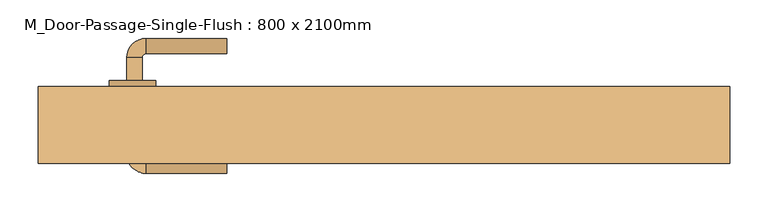
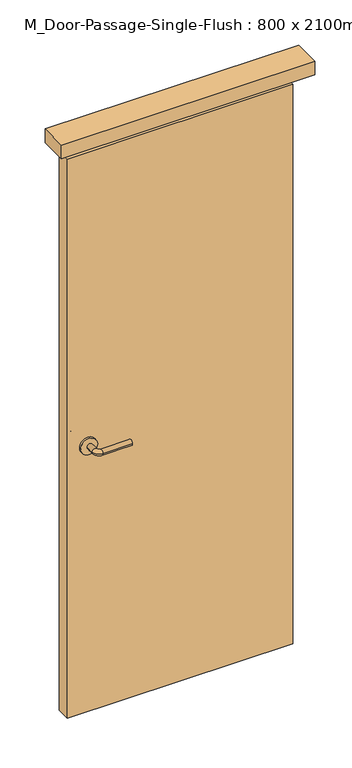
"""IFC4 building model written with IfcOpenShell, lengths in millimetres: door geometry, M_Door-Passage-Single-Flush : 800 x 2100mm."""

from ifc_helpers import new_model, si_unit, point, frame, frame_2d, origin, origin_with_axes, place, context, project, spatial, polyline, circle_curve, ellipse_curve, trimmed, segment, composite_curve, outline, extrude, source, transform, mapped, element, save
from ifc_brep_helpers import plane_surface, cylinder_surface, revolved_surface, advanced_brep


def m_door_passage_single_flush_800_x_2100mm_229ee9c9(model_context):
    return source(origin(), model_context, "Body", "SolidModel", [
        advanced_brep(
        [(-334.990625, -26.65, 1000.0), (-314.990625, -26.65, 1000.0), (-314.990625, -56.65, 1000.0), (-334.990625, -56.65, 1000.0), (-309.990625, -61.65, 1000.0), (-309.990625, -81.65, 1000.0), (-204.990625, -81.65, 1000.0), (-204.990625, -61.65, 1000.0)],
        [
            (0, 1, circle_curve(frame((-324.990625, -26.65, 1000.0), z_axis=(0.0, 1.0, 0.0), x_axis=(1.0, 0.0, 0.0)), 10.0)),
            (1, 0, circle_curve(frame((-324.990625, -26.65, 1000.0), z_axis=(0.0, 1.0, 0.0), x_axis=(1.0, 0.0, 0.0)), 10.0)),
            (1, 2),
            (2, 3, circle_curve(frame((-324.990625, -56.65, 1000.0), z_axis=(0.0, 1.0, 0.0), x_axis=(1.0, 0.0, 0.0)), 10.0)),
            (3, 0),
            (3, 2, circle_curve(frame((-324.990625, -56.65, 1000.0), z_axis=(0.0, 1.0, 0.0), x_axis=(1.0, 0.0, 0.0)), 10.0)),
            (4, 5, circle_curve(frame((-309.990625, -71.65, 1000.0), z_axis=(-1.0, 0.0, 0.0), x_axis=(0.0, 1.0, 0.0)), 10.0)),
            (5, 3, circle_curve(frame((-309.990625, -56.65, 1000.0), z_axis=(0.0, 0.0, -1.0), x_axis=(-1.0, 0.0, 0.0)), 25.0)),
            (2, 4, circle_curve(frame((-309.990625, -56.65, 1000.0), z_axis=(0.0, 0.0, 1.0), x_axis=(-1.0, 0.0, 0.0)), 5.0)),
            (5, 4, circle_curve(frame((-309.990625, -71.65, 1000.0), z_axis=(-1.0, 0.0, 0.0), x_axis=(0.0, 1.0, 0.0)), 10.0)),
            (6, 7, circle_curve(frame((-204.990625, -71.65, 1000.0), z_axis=(1.0, 0.0, 0.0), x_axis=(0.0, 1.0, 0.0)), 10.0)),
            (7, 6, circle_curve(frame((-204.990625, -71.65, 1000.0), z_axis=(1.0, 0.0, 0.0), x_axis=(0.0, 1.0, 0.0)), 10.0)),
            (4, 7),
            (6, 5),
        ],
        [
            plane_surface(frame((-324.990625, -26.65, 1000.0), z_axis=(0.0, 1.0, 0.0), x_axis=(0.0, 0.0, 1.0))),
            cylinder_surface(frame((-324.990625, -26.65, 1000.0), z_axis=(0.0, 1.0, 0.0), x_axis=(1.0, 0.0, 0.0)), 10.0),
            revolved_surface(trimmed(ellipse_curve(frame((-324.990625, -56.65, 1000.0), z_axis=(0.0, -1.0, 0.0), x_axis=(1.0, 0.0, 0.0)), 10.0, 10.0), [point((-334.990625, -56.65, 1000.0))], [point((-314.990625, -56.65, 1000.0))], True, "CARTESIAN"), (-309.990625, -56.65, 1000.0), (0.0, 0.0, -1.0)),
            revolved_surface(trimmed(ellipse_curve(frame((-324.990625, -56.65, 1000.0), z_axis=(0.0, -1.0, 0.0), x_axis=(1.0, 0.0, 0.0)), 10.0, 10.0), [point((-314.990625, -56.65, 1000.0))], [point((-334.990625, -56.65, 1000.0))], True, "CARTESIAN"), (-309.990625, -56.65, 1000.0), (0.0, 0.0, -1.0)),
            plane_surface(frame((-204.990625, -71.65, 1000.0), z_axis=(1.0, 0.0, 0.0), x_axis=(0.0, 0.0, 1.0))),
            cylinder_surface(frame((-309.990625, -71.65, 1000.0), z_axis=(-1.0, 0.0, 0.0), x_axis=(0.0, 1.0, 0.0)), 10.0),
        ],
        [
            (0, [[1, 2]]),
            (1, [[3, 4, 5, -2]]),
            (1, [[-5, 6, -3, -1]]),
            (2, [[7, 8, -4, 9]]),
            (3, [[10, -9, -6, -8]]),
            (4, [[11, 12]]),
            (5, [[13, -11, 14, -7]]),
            (5, [[-14, -12, -13, -10]]),
        ],
    ),
        extrude(outline(composite_curve([segment(trimmed(circle_curve(frame_2d((1000.0, -327.490625)), 30.0), [point((1000.0, -357.490625))], [point((1000.0, -297.490625))], False, "CARTESIAN"), True, "CONTINUOUS"), segment(trimmed(circle_curve(frame_2d((1000.0, -327.490625)), 30.0), [point((1000.0, -297.490625))], [point((1000.0, -357.490625))], False, "CARTESIAN"), True, "CONTINUOUS")], self_intersect=False)), frame((0.0, -26.65, 0.0), z_axis=(0.0, 1.0, 0.0), x_axis=(0.0, 0.0, 1.0)), (0.0, 0.0, 1.0), 8.0),
        advanced_brep(
        [(-334.990625, 39.35, 1000.0), (-314.990625, 39.35, 1000.0), (-334.990625, 69.35, 1000.0), (-314.990625, 69.35, 1000.0), (-309.990625, 74.35, 1000.0), (-309.990625, 94.35, 1000.0), (-204.990625, 94.35, 1000.0), (-204.990625, 74.35, 1000.0)],
        [
            (0, 1, circle_curve(frame((-324.990625, 39.35, 1000.0), z_axis=(0.0, -1.0, 0.0), x_axis=(1.0, 0.0, 0.0)), 10.0)),
            (1, 0, circle_curve(frame((-324.990625, 39.35, 1000.0), z_axis=(0.0, -1.0, 0.0), x_axis=(1.0, 0.0, 0.0)), 10.0)),
            (0, 2),
            (2, 3, circle_curve(frame((-324.990625, 69.35, 1000.0), z_axis=(0.0, -1.0, 0.0), x_axis=(1.0, 0.0, 0.0)), 10.0)),
            (3, 1),
            (3, 2, circle_curve(frame((-324.990625, 69.35, 1000.0), z_axis=(0.0, -1.0, 0.0), x_axis=(1.0, 0.0, 0.0)), 10.0)),
            (4, 3, circle_curve(frame((-309.990625, 69.35, 1000.0), z_axis=(0.0, 0.0, 1.0), x_axis=(-1.0, 0.0, 0.0)), 5.0)),
            (2, 5, circle_curve(frame((-309.990625, 69.35, 1000.0), z_axis=(0.0, 0.0, -1.0), x_axis=(-1.0, 0.0, 0.0)), 25.0)),
            (5, 4, circle_curve(frame((-309.990625, 84.35, 1000.0), z_axis=(-1.0, 0.0, 0.0), x_axis=(0.0, -1.0, 0.0)), 10.0)),
            (4, 5, circle_curve(frame((-309.990625, 84.35, 1000.0), z_axis=(-1.0, 0.0, 0.0), x_axis=(0.0, -1.0, 0.0)), 10.0)),
            (6, 7, circle_curve(frame((-204.990625, 84.35, 1000.0), z_axis=(1.0, 0.0, 0.0), x_axis=(0.0, -1.0, 0.0)), 10.0)),
            (7, 6, circle_curve(frame((-204.990625, 84.35, 1000.0), z_axis=(1.0, 0.0, 0.0), x_axis=(0.0, -1.0, 0.0)), 10.0)),
            (5, 6),
            (7, 4),
        ],
        [
            plane_surface(frame((-324.990625, 39.35, 1000.0), z_axis=(0.0, -1.0, 0.0), x_axis=(0.0, 0.0, 1.0))),
            cylinder_surface(frame((-324.990625, 39.35, 1000.0), z_axis=(0.0, -1.0, 0.0), x_axis=(1.0, 0.0, 0.0)), 10.0),
            revolved_surface(trimmed(ellipse_curve(frame((-324.990625, 69.35, 1000.0), z_axis=(0.0, -1.0, 0.0), x_axis=(1.0, 0.0, 0.0)), 10.0, 10.0), [point((-334.990625, 69.35, 1000.0))], [point((-314.990625, 69.35, 1000.0))], True, "CARTESIAN"), (-309.990625, 69.35, 1000.0), (0.0, 0.0, -1.0)),
            revolved_surface(trimmed(ellipse_curve(frame((-324.990625, 69.35, 1000.0), z_axis=(0.0, -1.0, 0.0), x_axis=(1.0, 0.0, 0.0)), 10.0, 10.0), [point((-314.990625, 69.35, 1000.0))], [point((-334.990625, 69.35, 1000.0))], True, "CARTESIAN"), (-309.990625, 69.35, 1000.0), (0.0, 0.0, -1.0)),
            plane_surface(frame((-204.990625, 84.35, 1000.0), z_axis=(1.0, 0.0, 0.0), x_axis=(0.0, 0.0, 1.0))),
            cylinder_surface(frame((-309.990625, 84.35, 1000.0), z_axis=(-1.0, 0.0, 0.0), x_axis=(0.0, -1.0, 0.0)), 10.0),
        ],
        [
            (0, [[1, 2]]),
            (1, [[-1, 3, 4, 5]]),
            (1, [[-2, -5, 6, -3]]),
            (2, [[7, -4, 8, 9]]),
            (3, [[-8, -6, -7, 10]]),
            (4, [[11, 12]]),
            (5, [[-9, 13, -12, 14]]),
            (5, [[-10, -14, -11, -13]]),
        ],
    ),
        extrude(outline(composite_curve([segment(trimmed(circle_curve(frame_2d((1000.0, -327.490625)), 30.0), [point((1000.0, -357.490625))], [point((1000.0, -297.490625))], False, "CARTESIAN"), True, "CONTINUOUS"), segment(trimmed(circle_curve(frame_2d((1000.0, -327.490625)), 30.0), [point((1000.0, -297.490625))], [point((1000.0, -357.490625))], False, "CARTESIAN"), True, "CONTINUOUS")], self_intersect=False)), frame((0.0, 31.35, 0.0), z_axis=(0.0, 1.0, 0.0), x_axis=(0.0, 0.0, 1.0)), (0.0, 0.0, 1.0), 8.0),
        extrude(outline(polyline([(400.0, -18.65), (-400.0, -18.65), (-400.0, 31.35), (400.0, 31.35), (400.0, -18.65)])), origin_with_axes(), (0.0, 0.0, 1.0), 2100.0),
        extrude(outline(polyline([(450.0, 31.35), (450.0, -68.65), (-450.0, -68.65), (-450.0, 31.35), (450.0, 31.35)])), frame((0.0, 0.0, 2149.2), z_axis=(0.0, 0.0, 1.0), x_axis=(1.0, 0.0, 0.0)), (0.0, 0.0, 1.0), 50.8),
    ])


if __name__ == "__main__":
    model = new_model("IFC4")
    model_context = context("Model", 3, world=origin())
    ifc_project = project(units=[si_unit("LENGTHUNIT", "METRE", prefix="MILLI")], contexts=[model_context])
    site = spatial("IfcSite", under=ifc_project)
    building = spatial("IfcBuilding", under=site)
    placement = place(None, origin())
    m_door_passage_single_flush_800_x_2100mm_shape = m_door_passage_single_flush_800_x_2100mm_229ee9c9(model_context)
    element("IfcDoor", 1, ObjectType="M_Door-Passage-Single-Flush : 800 x 2100mm", at=placement, inside=building, context=model_context, shape_type="MappedRepresentation", body=[
        mapped(m_door_passage_single_flush_800_x_2100mm_shape, transform((0.0, 0.0, 0.0), x_axis=(1.0, 0.0, 0.0), y_axis=(0.0, 1.0, 0.0), z_axis=(0.0, 0.0, 1.0))),
    ])
    save(model, "model.ifc")

# Revit data of these elements
# Type "M_Door-Passage-Single-Flush : 800 x 2100mm"
#   Type Mark = "46"
#   Assembly Code = "B2030200"
#   Analytic Construction = "Wooden"
#   Thickness = 50 mm
#   Thermal Resistance (R) = 0.455703 (m²·K)/W
#   Swing Angle [instance default] = 90.00°
#   Strike Height = 1000 mm
#   Rough Width [instance default] = 900 mm
#   Rough Height [instance default] = 2200 mm
#   MF Opening Height [instance default] = 100 mm
#   MF Opening Width [instance default] = 100 mm
#   Inset Calculate [instance default] = 105 mm
#   Masonry Inset [instance default] = 25 mm
#   Height = 2100 mm
#   Width = 800 mm
#   Heat Transfer Coefficient (U) = 2.19465 W/(m²·K)
#   Masonry Frame Depth = 100 mm
#   Masonry Frame [instance default] = yes
#   Function = 1
#   Dry Wall Frame [instance default] = no
#   Panel Material = Wood - Birch
#   Frame Material = Metal - Paint Finish - Grey
#   Door Handle Material = Aluminum
#   Visual Light Transmittance = 0
#   Solar Heat Gain Coefficient = 0
#   Wall Closure = (empty or 0)
# Element 1 (IfcDoor, "M_Door-Passage-Single-Flush : 800 x 2100mm")
#   Materials on its faces: "Aluminum", "Wood - Birch", "Metal - Paint Finish - Grey"
# Materials
#   "Wood - Birch": class "Wood", colour RGB 173 132 96, transparency 0, Cost = 0
#   "Metal - Paint Finish - Grey": class "Paint", colour RGB 178 178 178, transparency 0, Cost = 0
#   "Aluminum": class "Metal", colour RGB 244 245 246, transparency 0, Description = "Aluminum 6061", Cost = 0
